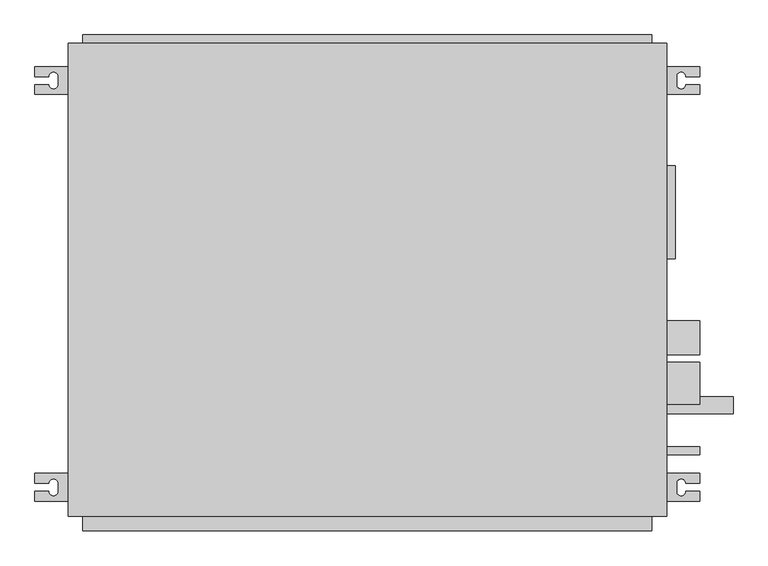
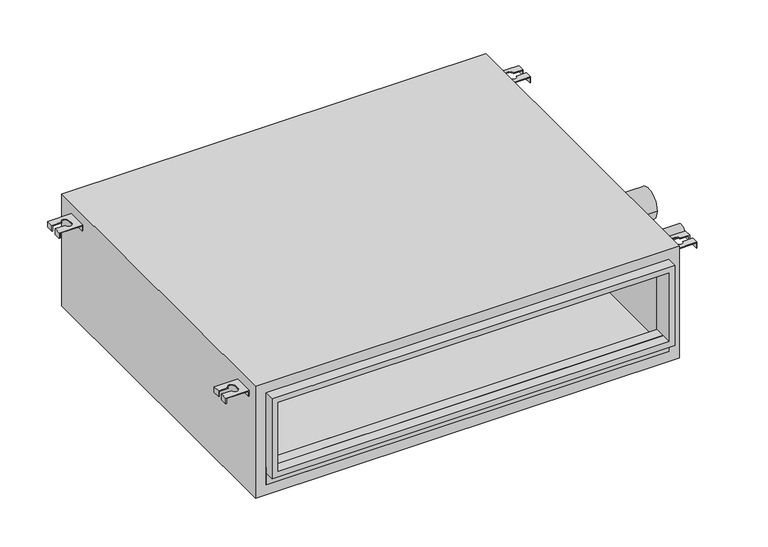
"""IFC4 building model written with IfcOpenShell, lengths in millimetres: proxy geometry, PEFY-P-NMAU-E_Medium_Static_Ducted : PEFY-P18NMAU-E."""

from ifc_helpers import new_model, si_unit, point, frame, frame_2d, origin, place, context, project, spatial, polyline, circle_curve, trimmed, segment, composite_curve, outline, extrude, source, transform, mapped, element, save
from ifc_brep_helpers import plane_surface, revolved_surface, advanced_brep


def mechanical_equipment_7e022f85(model_context):
    return source(origin(), model_context, "Body", "SolidModel", [
        advanced_brep(
        [(-510.074743, -231.05, 249.2375), (-510.074743, -246.05, 249.2375), (-489.068493, -246.05, 249.2375), (-475.068493, -246.05, 249.2375), (-475.068493, -258.05, 249.2375), (-489.068493, -258.05, 249.2375), (-510.074743, -258.05, 249.2375), (-510.074743, -273.05, 249.2375), (-460.068493, -273.05, 249.2375), (-460.068493, -231.05, 249.2375), (-510.074743, -231.05, 236.4972162), (-508.486743, -231.05, 236.4972162), (-508.486743, -246.05, 236.4972162), (-510.074743, -246.05, 236.4972162), (-508.486743, -273.05, 236.4972162), (-510.074743, -273.05, 236.4972162), (-510.074743, -258.05, 236.4972162), (-508.486743, -258.05, 236.4972162), (-460.068493, -231.05, 236.4972162), (-460.068493, -273.05, 236.4972162), (-461.656493, -273.05, 236.4972162), (-461.656493, -231.05, 236.4972162), (-508.486743, -246.05, 247.65), (-489.068493, -246.05, 247.65), (-508.486743, -231.05, 247.65), (-461.656493, -231.05, 247.65), (-508.486743, -258.05, 247.65), (-508.486743, -273.05, 247.65), (-489.068493, -258.05, 247.65), (-461.656493, -273.05, 247.65), (-475.068493, -258.05, 247.65), (-475.068493, -246.05, 247.65)],
        [
            (0, 1),
            (1, 2),
            (2, 3, circle_curve(frame((-482.068493, -246.05, 249.2375), z_axis=(0.0, 0.0, -1.0), x_axis=(1.0, 0.0, 0.0)), 7.0)),
            (3, 4),
            (4, 5, circle_curve(frame((-482.068493, -258.05, 249.2375), z_axis=(0.0, 0.0, -1.0), x_axis=(1.0, 0.0, 0.0)), 7.0)),
            (5, 6),
            (6, 7),
            (7, 8),
            (8, 9),
            (9, 0),
            (10, 11),
            (11, 12),
            (12, 13),
            (13, 10),
            (14, 15),
            (15, 16),
            (16, 17),
            (17, 14),
            (18, 19),
            (19, 20),
            (20, 21),
            (21, 18),
            (13, 1),
            (0, 10),
            (12, 22),
            (22, 23),
            (23, 2),
            (11, 24),
            (24, 22),
            (9, 18),
            (21, 25),
            (25, 24),
            (17, 26),
            (26, 27),
            (27, 14),
            (5, 28),
            (28, 26),
            (16, 6),
            (15, 7),
            (27, 29),
            (29, 20),
            (19, 8),
            (29, 25),
            (30, 31),
            (31, 23, circle_curve(frame((-482.068493, -246.05, 247.65), z_axis=(0.0, 0.0, 1.0), x_axis=(1.0, 0.0, 0.0)), 7.0)),
            (28, 30, circle_curve(frame((-482.068493, -258.05, 247.65), z_axis=(0.0, 0.0, 1.0), x_axis=(1.0, 0.0, 0.0)), 7.0)),
            (4, 30),
            (31, 3),
        ],
        [
            plane_surface(frame((-510.074743, -231.05, 249.2375), z_axis=(0.0, 0.0, 1.0), x_axis=(0.0, -1.0, 0.0))),
            plane_surface(frame((-510.074743, -231.05, 236.4972162), z_axis=(0.0, 0.0, -1.0), x_axis=(0.0, 1.0, 0.0))),
            plane_surface(frame((-510.074743, -231.05, 249.2375), z_axis=(-1.0, 0.0, 0.0), x_axis=(0.0, 0.0, -1.0))),
            plane_surface(frame((-510.074743, -246.05, 249.2375), z_axis=(0.0, -1.0, 0.0), x_axis=(0.0, 0.0, -1.0))),
            plane_surface(frame((-508.486743, -246.05, 249.2375), z_axis=(1.0, 0.0, 0.0), x_axis=(0.0, 0.0, -1.0))),
            plane_surface(frame((-508.486743, -231.05, 249.2375), z_axis=(0.0, 1.0, 0.0), x_axis=(0.0, 0.0, -1.0))),
            plane_surface(frame((-508.486743, -273.05, 249.2375), z_axis=(1.0, 0.0, 0.0), x_axis=(0.0, 0.0, -1.0))),
            plane_surface(frame((-508.486743, -258.05, 249.2375), z_axis=(0.0, 1.0, 0.0), x_axis=(0.0, 0.0, -1.0))),
            plane_surface(frame((-510.074743, -258.05, 249.2375), z_axis=(-1.0, 0.0, 0.0), x_axis=(0.0, 0.0, -1.0))),
            plane_surface(frame((-510.074743, -273.05, 249.2375), z_axis=(0.0, -1.0, 0.0), x_axis=(0.0, 0.0, -1.0))),
            plane_surface(frame((-461.656493, -231.05, 249.2375), z_axis=(-1.0, 0.0, 0.0), x_axis=(0.0, 0.0, -1.0))),
            plane_surface(frame((-460.068493, -273.05, 249.2375), z_axis=(1.0, 0.0, 0.0), x_axis=(0.0, 0.0, -1.0))),
            plane_surface(frame((-475.068493, -258.05, 247.65), z_axis=(0.0, 0.0, -1.0), x_axis=(0.0, 1.0, 0.0))),
            revolved_surface(polyline([(-475.068493, -258.05, 247.65), (-475.068493, -258.05, 249.2375)]), (-482.068493, -258.05, 247.65), (0.0, 0.0, -1.0)),
            revolved_surface(polyline([(-475.068493, -246.05, 247.65), (-475.068493, -246.05, 249.2375)]), (-482.068493, -246.05, 247.65), (0.0, 0.0, -1.0)),
            plane_surface(frame((-475.068493, -246.05, 249.2375), z_axis=(-1.0, 0.0, 0.0), x_axis=(0.0, 0.0, -1.0))),
        ],
        [
            (0, [[1, 2, 3, 4, 5, 6, 7, 8, 9, 10]]),
            (1, [[11, 12, 13, 14]]),
            (1, [[15, 16, 17, 18]]),
            (1, [[19, 20, 21, 22]]),
            (2, [[23, -1, 24, -14]]),
            (3, [[-2, -23, -13, 25, 26, 27]]),
            (4, [[-12, 28, 29, -25]]),
            (5, [[-10, 30, -22, 31, 32, -28, -11, -24]]),
            (6, [[-18, 33, 34, 35]]),
            (7, [[-6, 36, 37, -33, -17, 38]]),
            (8, [[39, -7, -38, -16]]),
            (9, [[-8, -39, -15, -35, 40, 41, -20, 42]]),
            (10, [[-21, -41, 43, -31]]),
            (11, [[-30, -9, -42, -19]]),
            (12, [[44, 45, -26, -29, -32, -43, -40, -34, -37, 46]]),
            (13, [[-5, 47, -46, -36]]),
            (14, [[-3, -27, -45, 48]]),
            (15, [[-4, -48, -44, -47]]),
        ],
    ),
        advanced_brep(
        [(490.050257, -231.05, 249.2375), (440.044007, -231.05, 249.2375), (440.044007, -273.05, 249.2375), (490.050257, -273.05, 249.2375), (490.050257, -258.05, 249.2375), (469.044007, -258.05, 249.2375), (455.044007, -258.05, 249.2375), (455.044007, -246.05, 249.2375), (469.044007, -246.05, 249.2375), (490.050257, -246.05, 249.2375), (490.050257, -231.05, 236.4972162), (490.050257, -246.05, 236.4972162), (488.462257, -246.05, 236.4972162), (488.462257, -231.05, 236.4972162), (488.462257, -273.05, 236.4972162), (488.462257, -258.05, 236.4972162), (490.050257, -258.05, 236.4972162), (490.050257, -273.05, 236.4972162), (440.044007, -231.05, 236.4972162), (441.632007, -231.05, 236.4972162), (441.632007, -273.05, 236.4972162), (440.044007, -273.05, 236.4972162), (469.044007, -246.05, 247.65), (488.462257, -246.05, 247.65), (488.462257, -231.05, 247.65), (441.632007, -231.05, 247.65), (488.462257, -273.05, 247.65), (488.462257, -258.05, 247.65), (469.044007, -258.05, 247.65), (441.632007, -273.05, 247.65), (455.044007, -258.05, 247.65), (455.044007, -246.05, 247.65)],
        [
            (0, 1),
            (1, 2),
            (2, 3),
            (3, 4),
            (4, 5),
            (5, 6, circle_curve(frame((462.044007, -258.05, 249.2375), z_axis=(0.0, 0.0, -1.0), x_axis=(-1.0, 0.0, 0.0)), 7.0)),
            (6, 7),
            (7, 8, circle_curve(frame((462.044007, -246.05, 249.2375), z_axis=(0.0, 0.0, -1.0), x_axis=(-1.0, 0.0, 0.0)), 7.0)),
            (8, 9),
            (9, 0),
            (10, 11),
            (11, 12),
            (12, 13),
            (13, 10),
            (14, 15),
            (15, 16),
            (16, 17),
            (17, 14),
            (18, 19),
            (19, 20),
            (20, 21),
            (21, 18),
            (10, 0),
            (9, 11),
            (8, 22),
            (22, 23),
            (23, 12),
            (23, 24),
            (24, 13),
            (24, 25),
            (25, 19),
            (18, 1),
            (14, 26),
            (26, 27),
            (27, 15),
            (4, 16),
            (27, 28),
            (28, 5),
            (3, 17),
            (2, 21),
            (20, 29),
            (29, 26),
            (25, 29),
            (30, 28, circle_curve(frame((462.044007, -258.05, 247.65), z_axis=(0.0, 0.0, 1.0), x_axis=(-1.0, 0.0, 0.0)), 7.0)),
            (22, 31, circle_curve(frame((462.044007, -246.05, 247.65), z_axis=(0.0, 0.0, 1.0), x_axis=(-1.0, 0.0, 0.0)), 7.0)),
            (31, 30),
            (30, 6),
            (7, 31),
        ],
        [
            plane_surface(frame((490.050257, -231.05, 249.2375), z_axis=(0.0, 0.0, 1.0), x_axis=(0.0, -1.0, 0.0))),
            plane_surface(frame((490.050257, -231.05, 236.4972162), z_axis=(0.0, 0.0, -1.0), x_axis=(0.0, 1.0, 0.0))),
            plane_surface(frame((490.050257, -231.05, 249.2375), z_axis=(1.0, 0.0, 0.0), x_axis=(0.0, 0.0, -1.0))),
            plane_surface(frame((490.050257, -246.05, 249.2375), z_axis=(0.0, -1.0, 0.0), x_axis=(0.0, 0.0, -1.0))),
            plane_surface(frame((488.462257, -246.05, 249.2375), z_axis=(-1.0, 0.0, 0.0), x_axis=(0.0, 0.0, -1.0))),
            plane_surface(frame((488.462257, -231.05, 249.2375), z_axis=(0.0, 1.0, 0.0), x_axis=(0.0, 0.0, -1.0))),
            plane_surface(frame((488.462257, -273.05, 249.2375), z_axis=(-1.0, 0.0, 0.0), x_axis=(0.0, 0.0, -1.0))),
            plane_surface(frame((488.462257, -258.05, 249.2375), z_axis=(0.0, 1.0, 0.0), x_axis=(0.0, 0.0, -1.0))),
            plane_surface(frame((490.050257, -258.05, 249.2375), z_axis=(1.0, 0.0, 0.0), x_axis=(0.0, 0.0, -1.0))),
            plane_surface(frame((490.050257, -273.05, 249.2375), z_axis=(0.0, -1.0, 0.0), x_axis=(0.0, 0.0, -1.0))),
            plane_surface(frame((441.632007, -231.05, 249.2375), z_axis=(1.0, 0.0, 0.0), x_axis=(0.0, 0.0, -1.0))),
            plane_surface(frame((440.044007, -273.05, 249.2375), z_axis=(-1.0, 0.0, 0.0), x_axis=(0.0, 0.0, -1.0))),
            plane_surface(frame((455.044007, -258.05, 247.65), z_axis=(0.0, 0.0, -1.0), x_axis=(0.0, 1.0, 0.0))),
            revolved_surface(polyline([(455.044007, -258.05, 247.65), (455.044007, -258.05, 249.2375)]), (462.044007, -258.05, 247.65), (0.0, 0.0, -1.0)),
            revolved_surface(polyline([(455.044007, -246.05, 247.65), (455.044007, -246.05, 249.2375)]), (462.044007, -246.05, 247.65), (0.0, 0.0, -1.0)),
            plane_surface(frame((455.044007, -246.05, 249.2375), z_axis=(1.0, 0.0, 0.0), x_axis=(0.0, 0.0, -1.0))),
        ],
        [
            (0, [[1, 2, 3, 4, 5, 6, 7, 8, 9, 10]]),
            (1, [[11, 12, 13, 14]]),
            (1, [[15, 16, 17, 18]]),
            (1, [[19, 20, 21, 22]]),
            (2, [[-11, 23, -10, 24]]),
            (3, [[25, 26, 27, -12, -24, -9]]),
            (4, [[-27, 28, 29, -13]]),
            (5, [[-23, -14, -29, 30, 31, -19, 32, -1]]),
            (6, [[33, 34, 35, -15]]),
            (7, [[36, -16, -35, 37, 38, -5]]),
            (8, [[-17, -36, -4, 39]]),
            (9, [[40, -21, 41, 42, -33, -18, -39, -3]]),
            (10, [[-31, 43, -41, -20]]),
            (11, [[-22, -40, -2, -32]]),
            (12, [[44, -37, -34, -42, -43, -30, -28, -26, 45, 46]]),
            (13, [[-38, -44, 47, -6]]),
            (14, [[48, -45, -25, -8]]),
            (15, [[-47, -46, -48, -7]]),
        ],
    ),
        advanced_brep(
        [(-510.074743, 339.0, 249.2375), (-460.068493, 339.0, 249.2375), (-460.068493, 381.0, 249.2375), (-510.074743, 381.0, 249.2375), (-510.074743, 366.0, 249.2375), (-489.068493, 366.0, 249.2375), (-475.068493, 366.0, 249.2375), (-475.068493, 354.0, 249.2375), (-489.068493, 354.0, 249.2375), (-510.074743, 354.0, 249.2375), (-510.074743, 339.0, 236.4972162), (-510.074743, 354.0, 236.4972162), (-508.486743, 354.0, 236.4972162), (-508.486743, 339.0, 236.4972162), (-508.486743, 381.0, 236.4972162), (-508.486743, 366.0, 236.4972162), (-510.074743, 366.0, 236.4972162), (-510.074743, 381.0, 236.4972162), (-460.068493, 339.0, 236.4972162), (-461.656493, 339.0, 236.4972162), (-461.656493, 381.0, 236.4972162), (-460.068493, 381.0, 236.4972162), (-489.068493, 354.0, 247.65), (-508.486743, 354.0, 247.65), (-508.486743, 339.0, 247.65), (-461.656493, 339.0, 247.65), (-508.486743, 381.0, 247.65), (-508.486743, 366.0, 247.65), (-489.068493, 366.0, 247.65), (-461.656493, 381.0, 247.65), (-475.068493, 366.0, 247.65), (-475.068493, 354.0, 247.65)],
        [
            (0, 1),
            (1, 2),
            (2, 3),
            (3, 4),
            (4, 5),
            (5, 6, circle_curve(frame((-482.068493, 366.0, 249.2375), z_axis=(0.0, 0.0, -1.0), x_axis=(1.0, 0.0, 0.0)), 7.0)),
            (6, 7),
            (7, 8, circle_curve(frame((-482.068493, 354.0, 249.2375), z_axis=(0.0, 0.0, -1.0), x_axis=(1.0, 0.0, 0.0)), 7.0)),
            (8, 9),
            (9, 0),
            (10, 11),
            (11, 12),
            (12, 13),
            (13, 10),
            (14, 15),
            (15, 16),
            (16, 17),
            (17, 14),
            (18, 19),
            (19, 20),
            (20, 21),
            (21, 18),
            (10, 0),
            (9, 11),
            (8, 22),
            (22, 23),
            (23, 12),
            (23, 24),
            (24, 13),
            (24, 25),
            (25, 19),
            (18, 1),
            (14, 26),
            (26, 27),
            (27, 15),
            (4, 16),
            (27, 28),
            (28, 5),
            (3, 17),
            (2, 21),
            (20, 29),
            (29, 26),
            (25, 29),
            (30, 28, circle_curve(frame((-482.068493, 366.0, 247.65), z_axis=(0.0, 0.0, 1.0), x_axis=(1.0, 0.0, 0.0)), 7.0)),
            (22, 31, circle_curve(frame((-482.068493, 354.0, 247.65), z_axis=(0.0, 0.0, 1.0), x_axis=(1.0, 0.0, 0.0)), 7.0)),
            (31, 30),
            (30, 6),
            (7, 31),
        ],
        [
            plane_surface(frame((-510.074743, 339.0, 249.2375), z_axis=(0.0, 0.0, 1.0), x_axis=(0.0, 1.0, 0.0))),
            plane_surface(frame((-510.074743, 339.0, 236.4972162), z_axis=(0.0, 0.0, -1.0), x_axis=(0.0, -1.0, 0.0))),
            plane_surface(frame((-510.074743, 339.0, 249.2375), z_axis=(-1.0, 0.0, 0.0), x_axis=(0.0, 0.0, -1.0))),
            plane_surface(frame((-510.074743, 354.0, 249.2375), z_axis=(0.0, 1.0, 0.0), x_axis=(0.0, 0.0, -1.0))),
            plane_surface(frame((-508.486743, 354.0, 249.2375), z_axis=(1.0, 0.0, 0.0), x_axis=(0.0, 0.0, -1.0))),
            plane_surface(frame((-508.486743, 339.0, 249.2375), z_axis=(0.0, -1.0, 0.0), x_axis=(0.0, 0.0, -1.0))),
            plane_surface(frame((-508.486743, 381.0, 249.2375), z_axis=(1.0, 0.0, 0.0), x_axis=(0.0, 0.0, -1.0))),
            plane_surface(frame((-508.486743, 366.0, 249.2375), z_axis=(0.0, -1.0, 0.0), x_axis=(0.0, 0.0, -1.0))),
            plane_surface(frame((-510.074743, 366.0, 249.2375), z_axis=(-1.0, 0.0, 0.0), x_axis=(0.0, 0.0, -1.0))),
            plane_surface(frame((-510.074743, 381.0, 249.2375), z_axis=(0.0, 1.0, 0.0), x_axis=(0.0, 0.0, -1.0))),
            plane_surface(frame((-461.656493, 339.0, 249.2375), z_axis=(-1.0, 0.0, 0.0), x_axis=(0.0, 0.0, -1.0))),
            plane_surface(frame((-460.068493, 381.0, 249.2375), z_axis=(1.0, 0.0, 0.0), x_axis=(0.0, 0.0, -1.0))),
            plane_surface(frame((-475.068493, 366.0, 247.65), z_axis=(0.0, 0.0, -1.0), x_axis=(0.0, -1.0, 0.0))),
            revolved_surface(polyline([(-475.068493, 366.0, 247.65), (-475.068493, 366.0, 249.2375)]), (-482.068493, 366.0, 247.65), (0.0, 0.0, -1.0)),
            revolved_surface(polyline([(-475.068493, 354.0, 247.65), (-475.068493, 354.0, 249.2375)]), (-482.068493, 354.0, 247.65), (0.0, 0.0, -1.0)),
            plane_surface(frame((-475.068493, 354.0, 249.2375), z_axis=(-1.0, 0.0, 0.0), x_axis=(0.0, 0.0, -1.0))),
        ],
        [
            (0, [[1, 2, 3, 4, 5, 6, 7, 8, 9, 10]]),
            (1, [[11, 12, 13, 14]]),
            (1, [[15, 16, 17, 18]]),
            (1, [[19, 20, 21, 22]]),
            (2, [[-11, 23, -10, 24]]),
            (3, [[25, 26, 27, -12, -24, -9]]),
            (4, [[-27, 28, 29, -13]]),
            (5, [[-23, -14, -29, 30, 31, -19, 32, -1]]),
            (6, [[33, 34, 35, -15]]),
            (7, [[36, -16, -35, 37, 38, -5]]),
            (8, [[-17, -36, -4, 39]]),
            (9, [[40, -21, 41, 42, -33, -18, -39, -3]]),
            (10, [[-31, 43, -41, -20]]),
            (11, [[-22, -40, -2, -32]]),
            (12, [[44, -37, -34, -42, -43, -30, -28, -26, 45, 46]]),
            (13, [[-38, -44, 47, -6]]),
            (14, [[48, -45, -25, -8]]),
            (15, [[-47, -46, -48, -7]]),
        ],
    ),
        advanced_brep(
        [(490.050257, 339.0, 249.2375), (490.050257, 354.0, 249.2375), (469.044007, 354.0, 249.2375), (455.044007, 354.0, 249.2375), (455.044007, 366.0, 249.2375), (469.044007, 366.0, 249.2375), (490.050257, 366.0, 249.2375), (490.050257, 381.0, 249.2375), (440.044007, 381.0, 249.2375), (440.044007, 339.0, 249.2375), (490.050257, 339.0, 236.4972162), (488.462257, 339.0, 236.4972162), (488.462257, 354.0, 236.4972162), (490.050257, 354.0, 236.4972162), (488.462257, 381.0, 236.4972162), (490.050257, 381.0, 236.4972162), (490.050257, 366.0, 236.4972162), (488.462257, 366.0, 236.4972162), (440.044007, 339.0, 236.4972162), (440.044007, 381.0, 236.4972162), (441.632007, 381.0, 236.4972162), (441.632007, 339.0, 236.4972162), (488.462257, 354.0, 247.65), (469.044007, 354.0, 247.65), (488.462257, 339.0, 247.65), (441.632007, 339.0, 247.65), (488.462257, 366.0, 247.65), (488.462257, 381.0, 247.65), (469.044007, 366.0, 247.65), (441.632007, 381.0, 247.65), (455.044007, 366.0, 247.65), (455.044007, 354.0, 247.65)],
        [
            (0, 1),
            (1, 2),
            (2, 3, circle_curve(frame((462.044007, 354.0, 249.2375), z_axis=(0.0, 0.0, -1.0), x_axis=(-1.0, 0.0, 0.0)), 7.0)),
            (3, 4),
            (4, 5, circle_curve(frame((462.044007, 366.0, 249.2375), z_axis=(0.0, 0.0, -1.0), x_axis=(-1.0, 0.0, 0.0)), 7.0)),
            (5, 6),
            (6, 7),
            (7, 8),
            (8, 9),
            (9, 0),
            (10, 11),
            (11, 12),
            (12, 13),
            (13, 10),
            (14, 15),
            (15, 16),
            (16, 17),
            (17, 14),
            (18, 19),
            (19, 20),
            (20, 21),
            (21, 18),
            (13, 1),
            (0, 10),
            (12, 22),
            (22, 23),
            (23, 2),
            (11, 24),
            (24, 22),
            (9, 18),
            (21, 25),
            (25, 24),
            (17, 26),
            (26, 27),
            (27, 14),
            (5, 28),
            (28, 26),
            (16, 6),
            (15, 7),
            (27, 29),
            (29, 20),
            (19, 8),
            (29, 25),
            (30, 31),
            (31, 23, circle_curve(frame((462.044007, 354.0, 247.65), z_axis=(0.0, 0.0, 1.0), x_axis=(-1.0, 0.0, 0.0)), 7.0)),
            (28, 30, circle_curve(frame((462.044007, 366.0, 247.65), z_axis=(0.0, 0.0, 1.0), x_axis=(-1.0, 0.0, 0.0)), 7.0)),
            (4, 30),
            (31, 3),
        ],
        [
            plane_surface(frame((490.050257, 339.0, 249.2375), z_axis=(0.0, 0.0, 1.0), x_axis=(0.0, 1.0, 0.0))),
            plane_surface(frame((490.050257, 339.0, 236.4972162), z_axis=(0.0, 0.0, -1.0), x_axis=(0.0, -1.0, 0.0))),
            plane_surface(frame((490.050257, 339.0, 249.2375), z_axis=(1.0, 0.0, 0.0), x_axis=(0.0, 0.0, -1.0))),
            plane_surface(frame((490.050257, 354.0, 249.2375), z_axis=(0.0, 1.0, 0.0), x_axis=(0.0, 0.0, -1.0))),
            plane_surface(frame((488.462257, 354.0, 249.2375), z_axis=(-1.0, 0.0, 0.0), x_axis=(0.0, 0.0, -1.0))),
            plane_surface(frame((488.462257, 339.0, 249.2375), z_axis=(0.0, -1.0, 0.0), x_axis=(0.0, 0.0, -1.0))),
            plane_surface(frame((488.462257, 381.0, 249.2375), z_axis=(-1.0, 0.0, 0.0), x_axis=(0.0, 0.0, -1.0))),
            plane_surface(frame((488.462257, 366.0, 249.2375), z_axis=(0.0, -1.0, 0.0), x_axis=(0.0, 0.0, -1.0))),
            plane_surface(frame((490.050257, 366.0, 249.2375), z_axis=(1.0, 0.0, 0.0), x_axis=(0.0, 0.0, -1.0))),
            plane_surface(frame((490.050257, 381.0, 249.2375), z_axis=(0.0, 1.0, 0.0), x_axis=(0.0, 0.0, -1.0))),
            plane_surface(frame((441.632007, 339.0, 249.2375), z_axis=(1.0, 0.0, 0.0), x_axis=(0.0, 0.0, -1.0))),
            plane_surface(frame((440.044007, 381.0, 249.2375), z_axis=(-1.0, 0.0, 0.0), x_axis=(0.0, 0.0, -1.0))),
            plane_surface(frame((455.044007, 366.0, 247.65), z_axis=(0.0, 0.0, -1.0), x_axis=(0.0, -1.0, 0.0))),
            revolved_surface(polyline([(455.044007, 366.0, 247.65), (455.044007, 366.0, 249.2375)]), (462.044007, 366.0, 247.65), (0.0, 0.0, -1.0)),
            revolved_surface(polyline([(455.044007, 354.0, 247.65), (455.044007, 354.0, 249.2375)]), (462.044007, 354.0, 247.65), (0.0, 0.0, -1.0)),
            plane_surface(frame((455.044007, 354.0, 249.2375), z_axis=(1.0, 0.0, 0.0), x_axis=(0.0, 0.0, -1.0))),
        ],
        [
            (0, [[1, 2, 3, 4, 5, 6, 7, 8, 9, 10]]),
            (1, [[11, 12, 13, 14]]),
            (1, [[15, 16, 17, 18]]),
            (1, [[19, 20, 21, 22]]),
            (2, [[23, -1, 24, -14]]),
            (3, [[-2, -23, -13, 25, 26, 27]]),
            (4, [[-12, 28, 29, -25]]),
            (5, [[-10, 30, -22, 31, 32, -28, -11, -24]]),
            (6, [[-18, 33, 34, 35]]),
            (7, [[-6, 36, 37, -33, -17, 38]]),
            (8, [[39, -7, -38, -16]]),
            (9, [[-8, -39, -15, -35, 40, 41, -20, 42]]),
            (10, [[-21, -41, 43, -31]]),
            (11, [[-30, -9, -42, -19]]),
            (12, [[44, 45, -26, -29, -32, -43, -40, -34, -37, 46]]),
            (13, [[-5, 47, -46, -36]]),
            (14, [[-3, -27, -45, 48]]),
            (15, [[-4, -48, -44, -47]]),
        ],
    ),
        extrude(outline(polyline([(417.819007, -295.275), (-437.843493, -295.275), (-437.843493, -273.05), (417.819007, -273.05), (417.819007, -295.275)])), frame((0.0, 0.0, 42.8625), z_axis=(0.0, 0.0, 1.0), x_axis=(1.0, 0.0, 0.0)), (0.0, 0.0, 1.0), 39.6875),
        extrude(outline(polyline([(249.2375, 417.819007), (249.2375, -437.843493), (69.85, -437.843493), (69.85, 417.819007), (249.2375, 417.819007)]), holes=[polyline([(82.55, 405.119007), (82.55, -425.143493), (236.5375, -425.143493), (236.5375, 405.119007), (82.55, 405.119007)])]), frame((0.0, -317.5, 0.0), z_axis=(0.0, 1.0, 0.0), x_axis=(0.0, 0.0, 1.0)), (0.0, 0.0, 1.0), 44.45),
        extrude(outline(polyline([(417.819007, 415.925), (-437.843493, 415.925), (-437.843493, 428.625), (417.819007, 428.625), (417.819007, 415.925)])), frame((0.0, 0.0, 42.8625), z_axis=(0.0, 0.0, 1.0), x_axis=(1.0, 0.0, 0.0)), (0.0, 0.0, 1.0), 206.375),
        extrude(outline(polyline([(271.4625, 440.044007), (271.4625, -460.068493), (20.6375, -460.068493), (20.6375, 440.044007), (271.4625, 440.044007)]), holes=[polyline([(42.8625, -437.843493), (249.2375, -437.843493), (249.2375, 417.819007), (42.8625, 417.819007), (42.8625, -437.843493)])]), frame((0.0, -295.275, 0.0), z_axis=(0.0, 1.0, 0.0), x_axis=(0.0, 0.0, 1.0)), (0.0, 0.0, 1.0), 711.2),
        extrude(outline(composite_curve([segment(trimmed(circle_curve(frame_2d((-26.9875, 109.5375)), 25.4), [point((-1.5875, 109.5375))], [point((-52.3875, 109.5375))], False, "CARTESIAN"), True, "CONTINUOUS"), segment(trimmed(circle_curve(frame_2d((-26.9875, 109.5375)), 25.4), [point((-52.3875, 109.5375))], [point((-1.5875, 109.5375))], False, "CARTESIAN"), True, "CONTINUOUS")], self_intersect=False)), frame((440.044007, 0.0, 0.0), z_axis=(1.0, 0.0, 0.0), x_axis=(0.0, 1.0, 0.0)), (0.0, 0.0, 1.0), 50.00625),
        extrude(outline(composite_curve([segment(trimmed(circle_curve(frame_2d((-128.5875, 171.45)), 12.7), [point((-115.8875, 171.45))], [point((-141.2875, 171.45))], False, "CARTESIAN"), True, "CONTINUOUS"), segment(trimmed(circle_curve(frame_2d((-128.5875, 171.45)), 12.7), [point((-141.2875, 171.45))], [point((-115.8875, 171.45))], False, "CARTESIAN"), True, "CONTINUOUS")], self_intersect=False)), frame((440.044007, 0.0, 0.0), z_axis=(1.0, 0.0, 0.0), x_axis=(0.0, 1.0, 0.0)), (0.0, 0.0, 1.0), 100.0125),
        extrude(outline(composite_curve([segment(trimmed(circle_curve(frame_2d((-95.25, 230.1875)), 31.75), [point((-63.5, 230.1875))], [point((-127.0, 230.1875))], False, "CARTESIAN"), True, "CONTINUOUS"), segment(trimmed(circle_curve(frame_2d((-95.25, 230.1875)), 31.75), [point((-127.0, 230.1875))], [point((-63.5, 230.1875))], False, "CARTESIAN"), True, "CONTINUOUS")], self_intersect=False)), frame((440.044007, 0.0, 0.0), z_axis=(1.0, 0.0, 0.0), x_axis=(0.0, 1.0, 0.0)), (0.0, 0.0, 1.0), 50.00625),
        extrude(outline(composite_curve([segment(trimmed(circle_curve(frame_2d((-196.85, 104.775)), 6.35), [point((-190.5, 104.775))], [point((-203.2, 104.775))], False, "CARTESIAN"), True, "CONTINUOUS"), segment(trimmed(circle_curve(frame_2d((-196.85, 104.775)), 6.35), [point((-203.2, 104.775))], [point((-190.5, 104.775))], False, "CARTESIAN"), True, "CONTINUOUS")], self_intersect=False)), frame((440.044007, 0.0, 0.0), z_axis=(1.0, 0.0, 0.0), x_axis=(0.0, 1.0, 0.0)), (0.0, 0.0, 1.0), 50.00625),
        extrude(outline(polyline([(452.744007, 231.84375), (452.744007, 92.14375), (440.044007, 92.14375), (440.044007, 231.84375), (452.744007, 231.84375)])), frame((0.0, 0.0, 42.8625), z_axis=(0.0, 0.0, 1.0), x_axis=(1.0, 0.0, 0.0)), (0.0, 0.0, 1.0), 187.325),
    ])


if __name__ == "__main__":
    model = new_model("IFC4")
    model_context = context("Model", 3, world=origin())
    ifc_project = project(units=[si_unit("LENGTHUNIT", "METRE", prefix="MILLI")], contexts=[model_context])
    site = spatial("IfcSite", under=ifc_project)
    building = spatial("IfcBuilding", under=site)
    placement = place(None, origin())
    mechanical_equipment_shape = mechanical_equipment_7e022f85(model_context)
    element("IfcBuildingElementProxy", 1, Name="PEFY-P-NMAU-E_Medium_Static_Ducted : PEFY-P18NMAU-E", ObjectType="PEFY-P-NMAU-E_Medium_Static_Ducted : PEFY-P18NMAU-E", at=placement, inside=building, context=model_context, shape_type="MappedRepresentation", body=[
        mapped(mechanical_equipment_shape, transform((0.0, 0.0, 0.0), x_axis=(1.0, 0.0, 0.0), y_axis=(0.0, 1.0, 0.0), z_axis=(0.0, 0.0, 1.0))),
    ])
    save(model, "model.ifc")

# Revit data of these elements
# Type "PEFY-P-NMAU-E_Medium_Static_Ducted : PEFY-P18NMAU-E"
#   Wiring (Min.size of wire) = "1/8"
#   Wiring (Amperage of wire breaker) = "15 A"
#   Voltage Options = "208/230 VAC"
#   Unit Weight (LBS) = "58"
#   Temperature set range Remote controller Heating = "63 to 83 F"
#   Temperature set range Remote controller Cooling = "67 to 86 F"
#   Subcategory = "HVAC"
#   Specification URL = ""
#   Sound Pressure Levels (dB(A)) = "26,28,29"
#   SmartBIM Object Created By = "Reed Construction Data"
#   Single Phase = "X"
#   Refrigerant control device = "LEV"
#   Protection devices = "Fuse"
#   Power input Heating = "0.09 kW"
#   Power input Cooling = "0.11 kW"
#   Moter Type = "DC blushless motor"
#   Moter Output = "0.085 kW"
#   Model = "PEFY-P18NMAU-E"
#   Manufacturer URL = ""
#   Manufacturer = "Mitsubishi Electric"
#   Insulation material = "EPS, Polyethylene foam, Urethane foam"
#   Installation URL = ""
#   Heating Capacity (kcal/h) = "5,100"
#   Heating Capacity (kW) = "5.9"
#   Heat exchanger = "Cross fin(Aluminium fin and copper tube)"
#   Frequency = "60 Hz"
#   Fan Type x Quantity = "Sirocco fan x 1"
#   E.S.P(mmH2O) = "3.6,5.1,7.1,10.2,15.3"
#   E.S.P(Pa) = "35,50,70,100,150"
#   E.S.P(In. W.G.) = "0.14,0.20,0.28,0.40,0.60"
#   Driving mechanism = "Direct-driven by motor"
#   Current Heating = "0.66 A"
#   Current Cooling = "0.77 A"
#   Cooling Capacity (kcal/h) = "4,600"
#   Cooling Capacity (kW) = "5.3"
#   Connectable outdoor unit = "R410A,R22 CITY MULTI"
#   Assembly Code = "D3050200"
#   Airflow rate(Low-Mid-High) (m3/min) = "6.0,7.5,8.5"
#   Airflow rate(Low-Mid-High) (cfm) = "212,265,300"
#   Airflow rate(Low-Mid-High) (L/s) = "100,125,142"
#   Air Filter = "PP Honeycomb fabric"
#   95 CSI = "15760"
#   04 CSI = "23 82 19"
#   Width = 2' - 11 7/16"
#   Voltage = 208 V
#   Unit Supply Airflow [instance default] = 0 CFM
#   Unit Return Airflow [instance default] = 0 CFM
#   SmartBIM Object Version = 3
#   Refrigerant Pipe Liquid = 0' - 0 1/4"
#   Refrigerant Pipe Gas = 0' - 0 1/2"
#   Refirigerant Pipe diameter (Liquid) = 0' - 0 1/4"
#   Refirigerant Pipe diameter (Gas) = 0' - 0 1/2"
#   Phase = 1
#   Nominal Heating Capacity = 20000.0 Btu/h
#   Nominal Cooling Capacity = 18000.0 Btu/h
#   Minimum Circuit Current = 1.56 A
#   Maximum Overcurrent Protection = 15 A
#   Hertz = 60
#   Height = 0' - 9 7/8"
#   Drain piping diameter = 0' - 1 1/4"
#   Drain Pump = 0' - 1"
#   Depth = 2' - 4 7/8"
#   Default Elevation = 4' - 0"
#   Back Air Inlet Width = 2' - 9 11/16"
#   Back Air Inlet Height = 0' - 8 1/8"
#   Apparent Load = 0 VA
#   Air Outlet Width = 2' - 9 11/16"
#   Air Outlet Height = 0' - 7 1/16"
#   Sound Pressure Levels @ Mid Airflow (dBA) = 32
#   Sound Pressure Levels @ Low Airflow (dBA) = 28
#   Sound Pressure Levels @ High Airflow (dBA) = 35
#   Number of Poles = 2
#   Unit = Metal - Steel Satin
#   Load Classification = Other
#   Back Air Inlet = Grille
# Element 1 (IfcBuildingElementProxy, "PEFY-P-NMAU-E_Medium_Static_Ducted : PEFY-P18NMAU-E")
#   Unit Supply Airflow = 600 CFM
#   Materials on its faces: "Metal - Steel Satin", "Grille"
# Materials
#   "Metal - Steel Satin": class "Metal", colour RGB 189 187 185, transparency 0
#   "Grille": class "Miscellaneous", colour RGB 0 0 0, transparency 0
